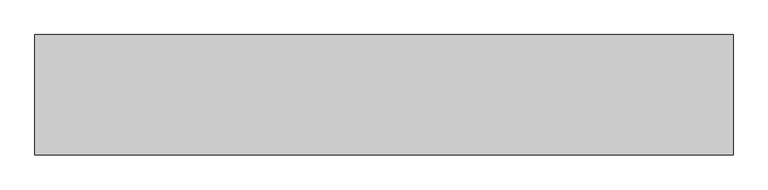
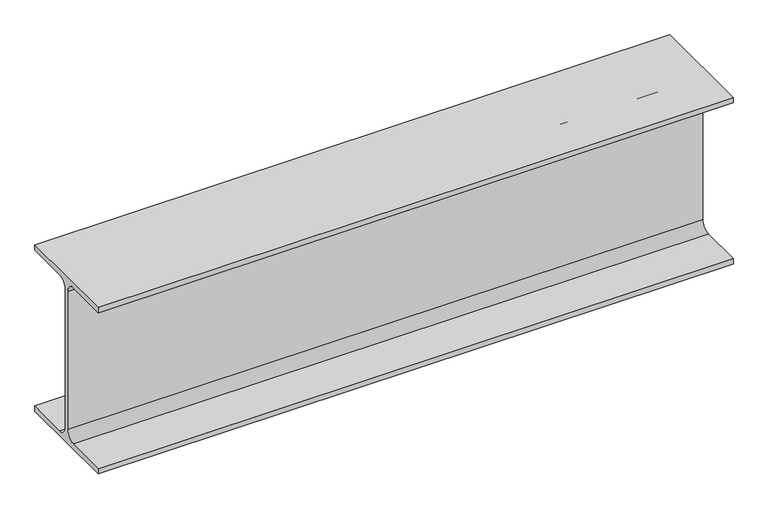
"""IFC4 building model written with IfcOpenShell, lengths in millimetres: beam geometry, 0912_Steel Framing_H-KSD3502 : H_SB_ASB_H-482x300x11x15."""

from ifc_helpers import new_model, si_unit, point, frame, frame_2d, origin, place, context, project, spatial, polyline, circle_curve, trimmed, segment, composite_curve, outline, extrude, source, transform, mapped, element, save


def beam_b23d1c7d(model_context):
    return source(origin(), model_context, "Body", "SweptSolid", [
        extrude(outline(composite_curve([segment(polyline([(150.0, -226.0), (150.0, -241.0), (-150.0, -241.0), (-150.0, -226.0), (-31.5, -226.0)]), True, "CONTINUOUS"), segment(trimmed(circle_curve(frame_2d((-31.5, -200.0)), 26.0), [point((-31.5, -226.0))], [point((-5.5, -200.0))], True, "CARTESIAN"), True, "CONTINUOUS"), segment(polyline([(-5.5, -200.0), (-5.5, 200.0)]), True, "CONTINUOUS"), segment(trimmed(circle_curve(frame_2d((-31.5, 200.0)), 26.0), [point((-5.5, 200.0))], [point((-31.5, 226.0))], True, "CARTESIAN"), True, "CONTINUOUS"), segment(polyline([(-31.5, 226.0), (-150.0, 226.0), (-150.0, 241.0), (150.0, 241.0), (150.0, 226.0), (31.5, 226.0)]), True, "CONTINUOUS"), segment(trimmed(circle_curve(frame_2d((31.5, 200.0)), 26.0), [point((31.5, 226.0))], [point((5.5, 200.0))], True, "CARTESIAN"), True, "CONTINUOUS"), segment(polyline([(5.5, 200.0), (5.5, -200.0)]), True, "CONTINUOUS"), segment(trimmed(circle_curve(frame_2d((31.5, -200.0)), 26.0), [point((5.5, -200.0))], [point((31.5, -226.0))], True, "CARTESIAN"), True, "CONTINUOUS"), segment(polyline([(31.5, -226.0), (150.0, -226.0)]), True, "CONTINUOUS")], self_intersect=False)), frame((-870.3, 0.0, 0.0), z_axis=(1.0, 0.0, 0.0), x_axis=(0.0, 1.0, 0.0)), (0.0, 0.0, 1.0), 1740.6),
    ])


if __name__ == "__main__":
    model = new_model("IFC4")
    model_context = context("Model", 3, world=origin())
    ifc_project = project(units=[si_unit("LENGTHUNIT", "METRE", prefix="MILLI")], contexts=[model_context])
    site = spatial("IfcSite", under=ifc_project)
    building = spatial("IfcBuilding", under=site)
    placement = place(None, origin())
    beam_shape = beam_b23d1c7d(model_context)
    element("IfcBeam", 1, ObjectType="0912_Steel Framing_H-KSD3502 : H_SB_ASB_H-482x300x11x15", at=placement, inside=building, context=model_context, shape_type="MappedRepresentation", body=[
        mapped(beam_shape, transform((0.0, 0.0, 0.0), x_axis=(1.0, 0.0, 0.0), y_axis=(0.0, 1.0, 0.0), z_axis=(0.0, 0.0, 1.0))),
    ])
    save(model, "model.ifc")

# Revit data of these elements
# Type "0912_Steel Framing_H-KSD3502 : H_SB_ASB_H-482x300x11x15"
#   H_WM Code_1 = "S01AA001-00001 | Main Steel Structure Fabrication Work | Shelter/Building | Heavy Steel - Standard (Weight≥90KG/M) | Material: (   )"
#   H_WM Code_2 = "S03AA027-00001 | Main Steel Structure Erection Work | Shelter/Building | Heavy Steel (Weight≥90KG/M) | Material: (   )"
#   H_WM Code_3 = "S01AA010-00001 | Main Steel Structure Fabrication Work | Shelter/Building | Steel Painting/Coating | for Non-Fireproofed Steel Surface, Surface Preparation, Primer, Second & Final Coat | Material: (   )"
#   H_Q'ty Cal Type Tag = "SB-Q2"
#   Width = 30.0 cm
#   Web Thickness = 1.1 cm
#   Web Fillet = 2.6 cm
#   Warping Constant = 3680000.0 cm⁶
#   W = 0
#   Torsional Moment of Inertia = 88.2192 cm⁴
#   Section Area = 145.5 cm²
#   Plastic Modulus weak axis = 695.0 cm³
#   Plastic Modulus strong axis = 2790.0 cm³
#   Perimeter = 2.10 m²/m
#   Nominal Weight = 114.00 kgf/m
#   Moment of Inertia weak axis = 6760.00 cm⁴
#   Moment of Inertia strong axis = 60400.00 cm⁴
#   Height = 48.2 cm
#   Flange Thickness = 1.5 cm
#   Elastic Modulus weak axis = 451.0 cm³
#   Elastic Modulus strong axis = 2500.0 cm³
#   Centroid Vertical = 24.1 cm
#   Centroid Horizontal = 15.0 cm
#   Ix = 604000000
#   Length [instance default] = 1.5240 m
#   Zx = 2790000
#   b = 0.3000 m
#   h = 0.4820 m
#   r = 0.0260 m
#   s = 0.0110 m
#   t = 0.0150 m
#   A = 0.01455 m²
#   Structural Material [instance default] = Steel, 45-345
#   Assembly Code = ""
# Element 1 (IfcBeam, "0912_Steel Framing_H-KSD3502 : H_SB_ASB_H-482x300x11x15")
#   Structural Material = none
# Materials
#   "Steel, 45-345": class "Metal", colour RGB 189 187 185, transparency 0, Description = "Steel 345 MPa", Cost = 0
